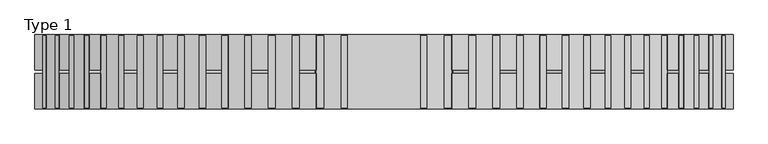
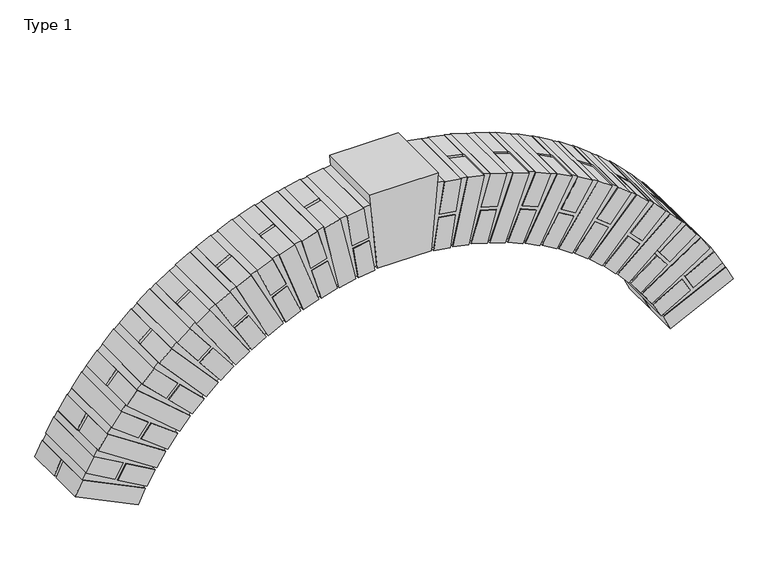
"""IFC4 building model written with IfcOpenShell, lengths in millimetres: proxy geometry, 00_GM_toog : Type 1."""

import ifcopenshell
import ifcopenshell.guid

model = None  # the IFC model being written
_history = None  # IfcOwnerHistory: only IFC2X3 demands one
_inside = {}  # id of a spatial element -> (the spatial element, [elements in it])
_under = {}  # id of a project, library or spatial element -> (it, [spatial elements below it])
_declared = {}  # id of a project -> (the project, [libraries it declares])
_typed = {}  # id of a type object -> (the type object, [elements of that type])
_made_of = {}  # id of a material, layer set ... -> (it, [elements and type objects made of it])


def new_model(schema):
    """Start an empty IFC model of exactly this schema.

    Asked for "IFC4X3", IfcOpenShell would pick the latest addendum, in which some entities
    have other attributes; the version numbers below select the first issue.
    IFC2X3 requires an IfcOwnerHistory on every rooted entity: one is made here for all.
    """
    global model, _history
    if schema == "IFC4X3":
        model = ifcopenshell.file(schema_version=(4, 3, 0, 0))
    else:
        model = ifcopenshell.file(schema=schema)
    _inside.clear()
    _under.clear()
    _declared.clear()
    _typed.clear()
    _made_of.clear()
    _history = None
    if model.schema == "IFC2X3":
        org = make("IfcOrganization", Name="unknown")
        user = make(
            "IfcPersonAndOrganization",
            ThePerson=make("IfcPerson", FamilyName="unknown"),
            TheOrganization=org,
        )
        app = make(
            "IfcApplication",
            ApplicationDeveloper=org,
            Version="unknown",
            ApplicationFullName="unknown",
            ApplicationIdentifier="unknown",
        )
        _history = make(
            "IfcOwnerHistory",
            OwningUser=user,
            OwningApplication=app,
            ChangeAction="ADDED",
            CreationDate=0,
        )
    return model


def make(cls, **values):
    """One entity of the class cls with the attributes given. An attribute that is None is left unset."""
    return model.create_entity(
        cls, **{name: value for name, value in values.items() if value is not None}
    )


def rooted(cls, **values):
    """An entity with a GlobalId (a new one), such as an element, a storey or a relation."""
    return make(cls, GlobalId=ifcopenshell.guid.new(), OwnerHistory=_history, **values)


def si_unit(unit_type, name, prefix=None):
    """IfcSIUnit, for example si_unit("LENGTHUNIT", "METRE", prefix="MILLI")."""
    return make("IfcSIUnit", UnitType=unit_type, Prefix=prefix, Name=name)


def assignment(units):
    """IfcUnitAssignment: the units of a project."""
    return None if units is None else make("IfcUnitAssignment", Units=units)


def point(xyz):
    """IfcCartesianPoint."""
    return None if xyz is None else make("IfcCartesianPoint", Coordinates=xyz)


def direction(xyz):
    """IfcDirection."""
    return None if xyz is None else make("IfcDirection", DirectionRatios=xyz)


def frame(location, z_axis=None, x_axis=None):
    """IfcAxis2Placement3D, a coordinate frame: its origin and axes. An axis left out is left unset."""
    return make(
        "IfcAxis2Placement3D",
        Location=point(location),
        Axis=direction(z_axis),
        RefDirection=direction(x_axis),
    )


def origin():
    """The frame at (0, 0, 0) with its axes left unset."""
    return frame((0.0, 0.0, 0.0))


def place(relative_to, where):
    """IfcLocalPlacement: puts the frame where relative to a parent placement (None: the world)."""
    return make(
        "IfcLocalPlacement", PlacementRelTo=relative_to, RelativePlacement=where
    )


def context(
    kind, dimensions, precision=None, world=None, true_north=None, identifier=None
):
    """IfcGeometricRepresentationContext, for example the 3D "Model" context."""
    return make(
        "IfcGeometricRepresentationContext",
        ContextIdentifier=identifier,
        ContextType=kind,
        CoordinateSpaceDimension=dimensions,
        Precision=precision,
        WorldCoordinateSystem=world,
        TrueNorth=true_north,
    )


def project(units=None, contexts=None):
    """IfcProject with its units and contexts."""
    return rooted(
        "IfcProject",
        Name="project",
        RepresentationContexts=contexts,
        UnitsInContext=assignment(units),
    )


def spatial(cls, under=None, at=None, **own):
    """A site, building, storey or space (cls), placed at a placement, below another one or the project."""
    s = rooted(cls, ObjectPlacement=at, **own)
    if under is not None:
        _under.setdefault(under.id(), (under, []))[1].append(s)
    return s


def polyline(points):
    """IfcPolyline through the points."""
    return make("IfcPolyline", Points=[point(p) for p in points])


def outline(outer, holes=None, kind="AREA"):
    """IfcArbitraryClosedProfileDef: a profile drawn as a closed curve; with holes, ...WithVoids."""
    if holes is None:
        return make("IfcArbitraryClosedProfileDef", ProfileType=kind, OuterCurve=outer)
    return make(
        "IfcArbitraryProfileDefWithVoids",
        ProfileType=kind,
        OuterCurve=outer,
        InnerCurves=holes,
    )


def extrude(swept, where, along, depth):
    """IfcExtrudedAreaSolid: the profile swept, set in the frame where, extruded along a direction by depth."""
    return make(
        "IfcExtrudedAreaSolid",
        SweptArea=swept,
        Position=where,
        ExtrudedDirection=direction(along),
        Depth=depth,
    )


def shape(context_of_items, identifier, shape_type, items):
    """IfcShapeRepresentation: the items that make up one representation, for example the "Body"."""
    return make(
        "IfcShapeRepresentation",
        ContextOfItems=context_of_items,
        RepresentationIdentifier=identifier,
        RepresentationType=shape_type,
        Items=items,
    )


def source(mapping_origin, context_of_items, identifier, shape_type, items):
    """IfcRepresentationMap: a shape defined once, which mapped items show again and again."""
    return make(
        "IfcRepresentationMap",
        MappingOrigin=mapping_origin,
        MappedRepresentation=shape(context_of_items, identifier, shape_type, items),
    )


def transform(
    local_origin,
    x_axis=None,
    y_axis=None,
    z_axis=None,
    scale=None,
    scale2=None,
    scale3=None,
    uniform=True,
):
    """IfcCartesianTransformationOperator3D, or its non-uniform kind. x_axis, y_axis, z_axis: its Axis1, 2, 3."""
    if uniform:
        return make(
            "IfcCartesianTransformationOperator3D",
            Axis1=direction(x_axis),
            Axis2=direction(y_axis),
            LocalOrigin=point(local_origin),
            Scale=scale,
            Axis3=direction(z_axis),
        )
    return make(
        "IfcCartesianTransformationOperator3DnonUniform",
        Axis1=direction(x_axis),
        Axis2=direction(y_axis),
        LocalOrigin=point(local_origin),
        Scale=scale,
        Axis3=direction(z_axis),
        Scale2=scale2,
        Scale3=scale3,
    )


def mapped(mapping_source, mapping_target):
    """IfcMappedItem: shows the shape of a source again, moved by a transform."""
    return make(
        "IfcMappedItem", MappingSource=mapping_source, MappingTarget=mapping_target
    )


def made_of(thing, what):
    """Note that an element or type object is made of a material, layer set ...; save() writes the relation."""
    if what is not None:
        _made_of.setdefault(what.id(), (what, []))[1].append(thing)
    return thing


def element(
    cls,
    number,
    at=None,
    inside=None,
    cuts=None,
    type_object=None,
    material=None,
    context=None,
    identifier="Body",
    shape_type=None,
    held_by="IfcProductDefinitionShape",
    body=None,
    shapes=None,
    **own,
):
    """One element of the class cls, such as IfcWall. Its Tag is "e" and its number.

    at: its placement. inside: the storey or other place that contains it. cuts: it is an
    opening in that element (IfcRelVoidsElement). A single representation is given by context,
    identifier, shape_type and body (its items); several are given by shapes. held_by: the class
    of the entity that holds the representations. save() writes the other relations.
    """
    e = rooted(cls, Tag="e%d" % number, ObjectPlacement=at, **own)
    if body is not None:
        shapes = [shape(context, identifier, shape_type, body)]
    if shapes is not None:
        e.Representation = make(held_by, Representations=shapes)
    if inside is not None:
        _inside.setdefault(inside.id(), (inside, []))[1].append(e)
    if cuts is not None:
        rooted(
            "IfcRelVoidsElement", RelatingBuildingElement=cuts, RelatedOpeningElement=e
        )
    if type_object is not None:
        _typed.setdefault(type_object.id(), (type_object, []))[1].append(e)
    return made_of(e, material)


def aggregate(whole, parts):
    """IfcRelAggregates: a whole, such as a stair, and the parts it consists of."""
    return rooted("IfcRelAggregates", RelatingObject=whole, RelatedObjects=parts)


def save(model, path):
    """Write the relations noted so far, then the file.

    IfcRelAggregates (storeys below a building ...), IfcRelContainedInSpatialStructure (elements
    in a storey), IfcRelDefinesByType, IfcRelAssociatesMaterial and IfcRelDeclares: one each for
    every whole, place, type object, material and project.
    """
    for whole, parts in _under.values():
        aggregate(whole, parts)
    for where, things in _inside.values():
        rooted(
            "IfcRelContainedInSpatialStructure",
            RelatedElements=things,
            RelatingStructure=where,
        )
    for kind, things in _typed.values():
        rooted("IfcRelDefinesByType", RelatedObjects=things, RelatingType=kind)
    for what, things in _made_of.values():
        rooted("IfcRelAssociatesMaterial", RelatedObjects=things, RelatingMaterial=what)
    for by, libraries in _declared.values():
        rooted("IfcRelDeclares", RelatingContext=by, RelatedDefinitions=libraries)
    model.write(path)


def type_1_0c07ca49(model_context):
    return source(origin(), model_context, "Body", "SweptSolid", [
        extrude(outline(polyline([(-45.6408721, 191.4818055), (-42.8894673, 170.9223699), (-141.6730221, 155.3721516), (-133.897913, 105.9803742), (-35.1143581, 121.5305924), (-31.8881677, 101.036053), (-232.700927, 82.4958258), (-234.4158083, 90.1571411), (-143.9996832, 104.390183), (-151.7747924, 153.7819605), (-244.0260363, 139.2600395), (-245.6920563, 146.7030645), (-45.6408721, 191.4818055)])), frame((0.0, 2.5, 0.0), z_axis=(0.0, 1.0, 0.0), x_axis=(0.0, 0.0, 1.0)), (0.0, 0.0, 1.0), 205.0),
        extrude(outline(polyline([(0.0, 50.0), (210.0, 50.0), (210.0, 0.0), (0.0, 0.0), (0.0, 50.0)])), frame((105.9803742, 210.0, -133.897913), z_axis=(0.15550218280693498, 0.0, 0.9878355486326045), x_axis=(0.0, -1.0, 0.0)), (0.0, 0.0, 1.0), 100.0),
        extrude(outline(polyline([(0.0, 50.0), (210.0, 50.0), (210.0, 0.0), (0.0, 0.0), (0.0, 50.0)])), frame((88.8399648, 210.0, -242.7832381), z_axis=(0.15550218280693498, 0.0, 0.9878355486326045), x_axis=(0.0, -1.0, 0.0)), (0.0, 0.0, 1.0), 100.0),
        extrude(outline(polyline([(210.0, 50.0), (210.0, 0.0), (110.0, 0.0), (110.0, 50.0), (210.0, 50.0)])), frame((194.4038505, 0.0, -261.4914261), z_axis=(0.2184312927282846, 0.0, 0.9758523302001438), x_axis=(0.0, 1.0, 0.0)), (0.0, 0.0, 1.0), 210.0),
        extrude(outline(polyline([(100.0, 50.0), (100.0, 0.0), (0.0, 0.0), (0.0, 50.0), (100.0, 50.0)])), frame((194.4038505, 0.0, -261.4914261), z_axis=(0.2184312927282846, 0.0, 0.9758523302001438), x_axis=(0.0, 1.0, 0.0)), (0.0, 0.0, 1.0), 210.0),
        extrude(outline(polyline([(-79.0011577, 328.483536), (-73.6449941, 308.4442712), (-169.6314476, 280.3978679), (-155.608246, 232.4046411), (-59.6217925, 260.4510444), (-53.8030292, 240.5368171), (-250.6000607, 196.486474), (-253.2799314, 203.8658279), (-165.42398, 229.5365694), (-179.4471816, 277.5297962), (-269.0862896, 251.3380319), (-271.689804, 258.5071292), (-79.0011577, 328.483536)])), frame((0.0, 2.5, 0.0), z_axis=(0.0, 1.0, 0.0), x_axis=(0.0, 0.0, 1.0)), (0.0, 0.0, 1.0), 205.0),
        extrude(outline(polyline([(0.0, 50.0), (210.0, 50.0), (210.0, 0.0), (0.0, 0.0), (0.0, 50.0)])), frame((232.4046411, 210.0, -155.608246), z_axis=(0.2804640326193317, 0.0, 0.9598645354459673), x_axis=(0.0, -1.0, 0.0)), (0.0, 0.0, 1.0), 100.0),
        extrude(outline(polyline([(0.0, 50.0), (210.0, 50.0), (210.0, 0.0), (0.0, 0.0), (0.0, 50.0)])), frame((201.4901661, 210.0, -261.4104336), z_axis=(0.2804640326193317, 0.0, 0.9598645354459673), x_axis=(0.0, -1.0, 0.0)), (0.0, 0.0, 1.0), 100.0),
        extrude(outline(polyline([(210.0, 50.0), (210.0, 0.0), (110.0, 0.0), (110.0, 50.0), (210.0, 50.0)])), frame((303.7977981, 0.0, -293.455382), z_axis=(0.34134584056160533, 0.0, 0.9399377730101558), x_axis=(0.0, 1.0, 0.0)), (0.0, 0.0, 1.0), 210.0),
        extrude(outline(polyline([(100.0, 50.0), (100.0, 0.0), (0.0, 0.0), (0.0, 50.0), (100.0, 50.0)])), frame((303.7977981, 0.0, -293.455382), z_axis=(0.34134584056160533, 0.0, 0.9399377730101558), x_axis=(0.0, 1.0, 0.0)), (0.0, 0.0, 1.0), 210.0),
        extrude(outline(polyline([(-129.5955556, 460.0988455), (-121.7224629, 440.9083522), (-213.3378444, 400.8256644), (-193.2965006, 355.0179737), (-101.681119, 395.1006614), (-93.3651981, 376.0932967), (-282.9194552, 307.2551682), (-286.5203712, 314.2315551), (-202.6652415, 350.9190515), (-222.7065854, 396.7267423), (-308.2636695, 359.294623), (-311.7619863, 366.072235), (-129.5955556, 460.0988455)])), frame((0.0, 2.5, 0.0), z_axis=(0.0, 1.0, 0.0), x_axis=(0.0, 0.0, 1.0)), (0.0, 0.0, 1.0), 205.0),
        extrude(outline(polyline([(0.0, 49.9999999), (210.0, 49.9999999), (210.0, 0.0), (0.0, 0.0), (0.0, 49.9999999)])), frame((355.0179737, 210.0, -193.2965006), z_axis=(0.40082687768196756, 0.0, 0.9161538157578809), x_axis=(0.0, -1.0, 0.0)), (0.0, 0.0, 1.0), 100.0),
        extrude(outline(polyline([(0.0, 50.0), (210.0, 50.0), (210.0, 0.0), (0.0, 0.0), (0.0, 50.0)])), frame((310.8363637, 210.0, -294.2806231), z_axis=(0.40082687768196756, 0.0, 0.9161538157578809), x_axis=(0.0, -1.0, 0.0)), (0.0, 0.0, 1.0), 100.0),
        extrude(outline(polyline([(210.0, 50.0), (210.0, 0.0), (110.0, 0.0), (110.0, 50.0), (210.0, 50.0)])), frame((408.2101175, 0.0, -339.136864), z_axis=(0.4586630534090749, 0.0, 0.8886102652104938), x_axis=(0.0, 1.0, 0.0)), (0.0, 0.0, 1.0), 210.0),
        extrude(outline(polyline([(100.0, 50.0), (100.0, 0.0), (0.0, 0.0), (0.0, 50.0), (100.0, 50.0)])), frame((408.2101175, 0.0, -339.136864), z_axis=(0.4586630534090749, 0.0, 0.8886102652104938), x_axis=(0.0, 1.0, 0.0)), (0.0, 0.0, 1.0), 210.0),
        extrude(outline(polyline([(-196.594427, 584.1695271), (-186.3335069, 566.142488), (-272.075522, 514.6807853), (-246.3446706, 471.8097777), (-160.6026555, 523.2714804), (-149.9259402, 505.482658), (-329.1291422, 412.9855408), (-333.5920562, 419.4445631), (-255.1127914, 466.5472186), (-280.8436427, 509.4182261), (-360.9157515, 461.3595579), (-365.2515057, 467.6345463), (-196.594427, 584.1695271)])), frame((0.0, 2.5, 0.0), z_axis=(0.0, 1.0, 0.0), x_axis=(0.0, 0.0, 1.0)), (0.0, 0.0, 1.0), 205.0),
        extrude(outline(polyline([(0.0, 50.0000001), (210.0, 50.0000001), (210.0, 0.0), (0.0, 0.0), (0.0, 50.0000001)])), frame((471.8097777, 210.0, -246.3446706), z_axis=(0.5146170271405577, 0.0, 0.8574201510210817), x_axis=(0.0, -1.0, 0.0)), (0.0, 0.0, 1.0), 100.0),
        extrude(outline(polyline([(0.0, 49.9999999), (210.0, 49.9999999), (210.0, 0.0), (0.0, 0.0), (0.0, 49.9999999)])), frame((415.0855159, 210.0, -340.8548065), z_axis=(0.5146170271405577, 0.0, 0.8574201510210817), x_axis=(0.0, -1.0, 0.0)), (0.0, 0.0, 1.0), 100.0),
        extrude(outline(polyline([(210.0, 50.0), (210.0, 0.0), (110.0, 0.0), (110.0, 50.0), (210.0, 50.0)])), frame((505.9286722, 0.0, -397.7867942), z_axis=(0.5684591822106966, 0.0, 0.8227114671379914), x_axis=(0.0, 1.0, 0.0)), (0.0, 0.0, 1.0), 210.0),
        extrude(outline(polyline([(100.0, 50.0), (100.0, 0.0), (0.0, 0.0), (0.0, 50.0), (100.0, 50.0)])), frame((505.9286722, 0.0, -397.7867942), z_axis=(0.5684591822106966, 0.0, 0.8227114671379914), x_axis=(0.0, 1.0, 0.0)), (0.0, 0.0, 1.0), 210.0),
        extrude(outline(polyline([(-278.8991351, 698.6610894), (-266.4186445, 682.093109), (-344.8813091, 620.0962521), (-313.8828807, 580.8649198), (-235.420216, 642.8617766), (-222.5577813, 626.5831948), (-388.4713826, 511.943842), (-393.7231125, 517.7795857), (-321.906603, 574.5250184), (-352.9050314, 613.7563507), (-426.1791551, 555.8591919), (-431.2812498, 561.5286604), (-278.8991351, 698.6610894)])), frame((0.0, 2.5, 0.0), z_axis=(0.0, 1.0, 0.0), x_axis=(0.0, 0.0, 1.0)), (0.0, 0.0, 1.0), 205.0),
        extrude(outline(polyline([(0.0, 50.0), (210.0, 50.0), (210.0, 0.0), (0.0, 0.0), (0.0, 50.0)])), frame((580.8649198, 210.0, -313.8828807), z_axis=(0.6199685681614698, 0.0, 0.784626646559889), x_axis=(0.0, -1.0, 0.0)), (0.0, 0.0, 1.0), 100.0),
        extrude(outline(polyline([(0.0, 50.0000001), (210.0, 50.0000001), (210.0, 0.0), (0.0, 0.0), (0.0, 50.0000001)])), frame((512.5281615, 210.0, -400.3692676), z_axis=(0.6199685681614698, 0.0, 0.784626646559889), x_axis=(0.0, -1.0, 0.0)), (0.0, 0.0, 1.0), 100.0),
        extrude(outline(polyline([(210.0, 50.0), (210.0, 0.0), (110.0, 0.0), (110.0, 50.0), (210.0, 50.0)])), frame((595.3510886, 0.0, -468.4434406), z_axis=(0.6689338074504708, 0.0, 0.7433219768376397), x_axis=(0.0, 1.0, 0.0)), (0.0, 0.0, 1.0), 210.0),
        extrude(outline(polyline([(100.0, 50.0), (100.0, 0.0), (0.0, 0.0), (0.0, 50.0), (100.0, 50.0)])), frame((595.3510886, 0.0, -468.4434406), z_axis=(0.6689338074504708, 0.0, 0.7433219768376397), x_axis=(0.0, 1.0, 0.0)), (0.0, 0.0, 1.0), 210.0),
        extrude(outline(polyline([(-375.1600602, 801.6961178), (-360.6646522, 786.8588753), (-430.5613481, 715.343479), (-394.8036499, 680.395131), (-324.9069541, 751.9105273), (-310.0697161, 737.4091197), (-459.9730918, 602.5073693), (-465.9275204, 607.6241406), (-401.951402, 673.0818479), (-437.7091002, 708.0301959), (-502.9837013, 641.243935), (-508.7684732, 646.2149166), (-375.1600602, 801.6961178)])), frame((0.0, 2.5, 0.0), z_axis=(0.0, 1.0, 0.0), x_axis=(0.0, 0.0, 1.0)), (0.0, 0.0, 1.0), 205.0),
        extrude(outline(polyline([(0.0, 100.0), (210.0, 100.0), (210.0, 0.0), (0.0, 0.0), (0.0, 100.0)])), frame((715.343479, 210.0, -430.5613481), z_axis=(-0.6989669587217563, 0.0, 0.7151539628746097), x_axis=(0.0, -1.0, 0.0)), (0.0, 0.0, 1.0), 50.0),
        extrude(outline(polyline([(0.0, 100.0), (210.0, 100.0), (210.0, 0.0), (0.0, 0.0), (0.0, 100.0)])), frame((636.5147996, 210.0, -507.6057961), z_axis=(-0.6989669587217563, 0.0, 0.7151539628746097), x_axis=(0.0, -1.0, 0.0)), (0.0, 0.0, 1.0), 50.0),
        extrude(outline(polyline([(0.0, 100.0), (210.0, 100.0), (210.0, 0.0), (0.0, 0.0), (0.0, 100.0)])), frame((675.0110323, 110.0, -549.9481866), z_axis=(-0.6517436105871354, 0.0, 0.7584393621502279), x_axis=(0.7584393621502279, 0.0, 0.6517436105871354)), (0.0, 0.0, 1.0), 50.0),
        extrude(outline(polyline([(0.0, 100.0), (210.0, 100.0), (210.0, 0.0), (0.0, 0.0), (0.0, 100.0)])), frame((675.0110323, 0.0, -549.9481866), z_axis=(-0.6517436105871354, 0.0, 0.7584393621502279), x_axis=(0.7584393621502279, 0.0, 0.6517436105871354)), (0.0, 0.0, 1.0), 50.0),
        extrude(outline(polyline([(-483.7987311, 891.5850605), (-467.5260991, 878.7218544), (-527.7106712, 798.8606168), (-487.7800524, 768.7683307), (-427.5954802, 848.6295684), (-411.0267377, 836.1431268), (-542.4617959, 683.1910761), (-549.0212836, 687.5049713), (-493.9346266, 760.6015881), (-533.8652454, 790.6938742), (-590.0699614, 716.1136617), (-596.4425527, 720.304643), (-483.7987311, 891.5850605)])), frame((0.0, 2.5, 0.0), z_axis=(0.0, 1.0, 0.0), x_axis=(0.0, 0.0, 1.0)), (0.0, 0.0, 1.0), 205.0),
        extrude(outline(polyline([(0.0, 99.9999999), (210.0, 99.9999999), (210.0, 0.0), (0.0, 0.0), (0.0, 99.9999999)])), frame((798.8606168, 210.0, -527.7106712), z_axis=(-0.6018457214896975, 0.0, 0.7986123762655734), x_axis=(0.0, -1.0, 0.0)), (0.0, 0.0, 1.0), 50.0),
        extrude(outline(polyline([(0.0, 100.0000001), (210.0, 100.0000001), (210.0, 0.0), (0.0, 0.0), (0.0, 100.0000001)])), frame((710.8326365, 210.0, -594.0498176), z_axis=(-0.6018457214896975, 0.0, 0.7986123762655734), x_axis=(0.0, -1.0, 0.0)), (0.0, 0.0, 1.0), 50.0),
        extrude(outline(polyline([(0.0, 100.0), (210.0, 100.0), (210.0, 0.0), (0.0, 0.0), (0.0, 100.0)])), frame((743.6022521, 110.0, -640.9645302), z_axis=(-0.5494780559199127, 0.0, 0.8355081484117753), x_axis=(0.8355081484117753, 0.0, 0.5494780559199127)), (0.0, 0.0, 1.0), 50.0),
        extrude(outline(polyline([(0.0, 100.0), (210.0, 100.0), (210.0, 0.0), (0.0, 0.0), (0.0, 100.0)])), frame((743.6022521, 0.0, -640.9645302), z_axis=(-0.5494780559199127, 0.0, 0.8355081484117753), x_axis=(0.8355081484117753, 0.0, 0.5494780559199127)), (0.0, 0.0, 1.0), 50.0),
        extrude(outline(polyline([(-603.0337079, 966.8539326), (-585.2506879, 956.175692), (-634.7362393, 869.2781649), (-591.2874757, 844.5353892), (-541.8019244, 931.4329163), (-523.7733689, 921.1661914), (-634.5848584, 752.6719241), (-641.6418437, 756.1122044), (-596.3479503, 835.6491039), (-639.7967139, 860.3918796), (-686.0099087, 779.24067), (-692.8658226, 782.582928), (-603.0337079, 966.8539326)])), frame((0.0, 2.5, 0.0), z_axis=(0.0, 1.0, 0.0), x_axis=(0.0, 0.0, 1.0)), (0.0, 0.0, 1.0), 205.0),
        extrude(outline(polyline([(0.0, 100.0000001), (210.0, 100.0000001), (210.0, 0.0), (0.0, 0.0), (0.0, 100.0000001)])), frame((869.2781649, 210.0, -634.7362393), z_axis=(-0.4948555135168874, 0.0, 0.8689752705007995), x_axis=(0.0, -1.0, 0.0)), (0.0, 0.0, 1.0), 50.0),
        extrude(outline(polyline([(0.0, 99.9999999), (210.0, 99.9999999), (210.0, 0.0), (0.0, 0.0), (0.0, 99.9999999)])), frame((773.4943526, 210.0, -689.2822652), z_axis=(-0.4948555135168874, 0.0, 0.8689752705007995), x_axis=(0.0, -1.0, 0.0)), (0.0, 0.0, 1.0), 50.0),
        extrude(outline(polyline([(0.0, 100.0), (210.0, 100.0), (210.0, 0.0), (0.0, 0.0), (0.0, 100.0)])), frame((800.0, 110.0, -740.0), z_axis=(-0.43820224719100825, 0.0, 0.8988764044943836), x_axis=(0.8988764044943836, 0.0, 0.43820224719100825)), (0.0, 0.0, 1.0), 50.0),
        extrude(outline(polyline([(0.0, 100.0), (210.0, 100.0), (210.0, 0.0), (0.0, 0.0), (0.0, 100.0)])), frame((800.0, 0.0, -740.0), z_axis=(-0.43820224719100825, 0.0, 0.8988764044943836), x_axis=(0.8988764044943836, 0.0, 0.43820224719100825)), (0.0, 0.0, 1.0), 50.0),
        extrude(outline(polyline([(-45.6408721, -191.4818055), (-245.6920563, -146.7030645), (-244.0260363, -139.2600395), (-151.7747924, -153.7819605), (-143.9996832, -104.390183), (-234.4158083, -90.1571411), (-232.700927, -82.4958258), (-31.8881677, -101.036053), (-35.1143581, -121.5305924), (-133.897913, -105.9803742), (-141.6730221, -155.3721516), (-42.8894673, -170.9223699), (-45.6408721, -191.4818055)])), frame((0.0, 2.5, 0.0), z_axis=(0.0, 1.0, 0.0), x_axis=(0.0, 0.0, 1.0)), (0.0, 0.0, 1.0), 205.0),
        extrude(outline(polyline([(0.0, -50.0), (0.0, 0.0), (210.0, 0.0), (210.0, -50.0), (0.0, -50.0)])), frame((-105.9803742, 210.0, -133.897913), z_axis=(-0.15550218280693498, 0.0, 0.9878355486326045), x_axis=(0.0, -1.0, 0.0)), (0.0, 0.0, 1.0), 100.0),
        extrude(outline(polyline([(0.0, -50.0), (0.0, 0.0), (210.0, 0.0), (210.0, -50.0), (0.0, -50.0)])), frame((-88.8399648, 210.0, -242.7832381), z_axis=(-0.15550218280693498, 0.0, 0.9878355486326045), x_axis=(0.0, -1.0, 0.0)), (0.0, 0.0, 1.0), 100.0),
        extrude(outline(polyline([(210.0, -50.0), (110.0, -50.0), (110.0, 0.0), (210.0, 0.0), (210.0, -50.0)])), frame((-194.4038505, 0.0, -261.4914261), z_axis=(-0.2184312927282846, 0.0, 0.9758523302001438), x_axis=(0.0, 1.0, 0.0)), (0.0, 0.0, 1.0), 210.0),
        extrude(outline(polyline([(100.0, -50.0), (0.0, -50.0), (0.0, 0.0), (100.0, 0.0), (100.0, -50.0)])), frame((-194.4038505, 0.0, -261.4914261), z_axis=(-0.2184312927282846, 0.0, 0.9758523302001438), x_axis=(0.0, 1.0, 0.0)), (0.0, 0.0, 1.0), 210.0),
        extrude(outline(polyline([(-79.0011577, -328.483536), (-271.689804, -258.5071292), (-269.0862896, -251.3380319), (-179.4471816, -277.5297962), (-165.42398, -229.5365694), (-253.2799314, -203.8658279), (-250.6000607, -196.486474), (-53.8030292, -240.5368171), (-59.6217925, -260.4510444), (-155.608246, -232.4046411), (-169.6314476, -280.3978679), (-73.6449941, -308.4442712), (-79.0011577, -328.483536)])), frame((0.0, 2.5, 0.0), z_axis=(0.0, 1.0, 0.0), x_axis=(0.0, 0.0, 1.0)), (0.0, 0.0, 1.0), 205.0),
        extrude(outline(polyline([(0.0, -50.0), (0.0, 0.0), (210.0, 0.0), (210.0, -50.0), (0.0, -50.0)])), frame((-232.4046411, 210.0, -155.608246), z_axis=(-0.2804640326193317, 0.0, 0.9598645354459673), x_axis=(0.0, -1.0, 0.0)), (0.0, 0.0, 1.0), 100.0),
        extrude(outline(polyline([(0.0, -50.0), (0.0, 0.0), (210.0, 0.0), (210.0, -50.0), (0.0, -50.0)])), frame((-201.4901661, 210.0, -261.4104336), z_axis=(-0.2804640326193317, 0.0, 0.9598645354459673), x_axis=(0.0, -1.0, 0.0)), (0.0, 0.0, 1.0), 100.0),
        extrude(outline(polyline([(210.0, -50.0), (110.0, -50.0), (110.0, 0.0), (210.0, 0.0), (210.0, -50.0)])), frame((-303.7977981, 0.0, -293.455382), z_axis=(-0.34134584056160533, 0.0, 0.9399377730101558), x_axis=(0.0, 1.0, 0.0)), (0.0, 0.0, 1.0), 210.0),
        extrude(outline(polyline([(100.0, -50.0), (0.0, -50.0), (0.0, 0.0), (100.0, 0.0), (100.0, -50.0)])), frame((-303.7977981, 0.0, -293.455382), z_axis=(-0.34134584056160533, 0.0, 0.9399377730101558), x_axis=(0.0, 1.0, 0.0)), (0.0, 0.0, 1.0), 210.0),
        extrude(outline(polyline([(-129.5955556, -460.0988455), (-311.7619863, -366.072235), (-308.2636695, -359.294623), (-222.7065854, -396.7267423), (-202.6652415, -350.9190515), (-286.5203712, -314.2315551), (-282.9194552, -307.2551682), (-93.3651981, -376.0932967), (-101.681119, -395.1006614), (-193.2965006, -355.0179737), (-213.3378444, -400.8256644), (-121.7224629, -440.9083522), (-129.5955556, -460.0988455)])), frame((0.0, 2.5, 0.0), z_axis=(0.0, 1.0, 0.0), x_axis=(0.0, 0.0, 1.0)), (0.0, 0.0, 1.0), 205.0),
        extrude(outline(polyline([(0.0, -49.9999999), (0.0, 0.0), (210.0, 0.0), (210.0, -49.9999999), (0.0, -49.9999999)])), frame((-355.0179737, 210.0, -193.2965006), z_axis=(-0.40082687768196756, 0.0, 0.9161538157578809), x_axis=(0.0, -1.0, 0.0)), (0.0, 0.0, 1.0), 100.0),
        extrude(outline(polyline([(0.0, -50.0), (0.0, 0.0), (210.0, 0.0), (210.0, -50.0), (0.0, -50.0)])), frame((-310.8363637, 210.0, -294.2806231), z_axis=(-0.40082687768196756, 0.0, 0.9161538157578809), x_axis=(0.0, -1.0, 0.0)), (0.0, 0.0, 1.0), 100.0),
        extrude(outline(polyline([(210.0, -50.0), (110.0, -50.0), (110.0, 0.0), (210.0, 0.0), (210.0, -50.0)])), frame((-408.2101175, 0.0, -339.136864), z_axis=(-0.4586630534090749, 0.0, 0.8886102652104938), x_axis=(0.0, 1.0, 0.0)), (0.0, 0.0, 1.0), 210.0),
        extrude(outline(polyline([(100.0, -50.0), (0.0, -50.0), (0.0, 0.0), (100.0, 0.0), (100.0, -50.0)])), frame((-408.2101175, 0.0, -339.136864), z_axis=(-0.4586630534090749, 0.0, 0.8886102652104938), x_axis=(0.0, 1.0, 0.0)), (0.0, 0.0, 1.0), 210.0),
        extrude(outline(polyline([(-196.594427, -584.1695271), (-365.2515057, -467.6345463), (-360.9157515, -461.3595579), (-280.8436427, -509.4182261), (-255.1127914, -466.5472186), (-333.5920562, -419.4445631), (-329.1291422, -412.9855408), (-149.9259402, -505.482658), (-160.6026555, -523.2714804), (-246.3446706, -471.8097777), (-272.075522, -514.6807853), (-186.3335069, -566.142488), (-196.594427, -584.1695271)])), frame((0.0, 2.5, 0.0), z_axis=(0.0, 1.0, 0.0), x_axis=(0.0, 0.0, 1.0)), (0.0, 0.0, 1.0), 205.0),
        extrude(outline(polyline([(0.0, -50.0000001), (0.0, 0.0), (210.0, 0.0), (210.0, -50.0000001), (0.0, -50.0000001)])), frame((-471.8097777, 210.0, -246.3446706), z_axis=(-0.5146170271405577, 0.0, 0.8574201510210817), x_axis=(0.0, -1.0, 0.0)), (0.0, 0.0, 1.0), 100.0),
        extrude(outline(polyline([(0.0, -49.9999999), (0.0, 0.0), (210.0, 0.0), (210.0, -49.9999999), (0.0, -49.9999999)])), frame((-415.0855159, 210.0, -340.8548065), z_axis=(-0.5146170271405577, 0.0, 0.8574201510210817), x_axis=(0.0, -1.0, 0.0)), (0.0, 0.0, 1.0), 100.0),
        extrude(outline(polyline([(210.0, -50.0), (110.0, -50.0), (110.0, 0.0), (210.0, 0.0), (210.0, -50.0)])), frame((-505.9286722, 0.0, -397.7867942), z_axis=(-0.5684591822106966, 0.0, 0.8227114671379914), x_axis=(0.0, 1.0, 0.0)), (0.0, 0.0, 1.0), 210.0),
        extrude(outline(polyline([(100.0, -50.0), (0.0, -50.0), (0.0, 0.0), (100.0, 0.0), (100.0, -50.0)])), frame((-505.9286722, 0.0, -397.7867942), z_axis=(-0.5684591822106966, 0.0, 0.8227114671379914), x_axis=(0.0, 1.0, 0.0)), (0.0, 0.0, 1.0), 210.0),
        extrude(outline(polyline([(-278.8991351, -698.6610894), (-431.2812498, -561.5286604), (-426.1791551, -555.8591919), (-352.9050314, -613.7563507), (-321.906603, -574.5250184), (-393.7231125, -517.7795857), (-388.4713826, -511.943842), (-222.5577813, -626.5831948), (-235.420216, -642.8617766), (-313.8828807, -580.8649198), (-344.8813091, -620.0962521), (-266.4186445, -682.093109), (-278.8991351, -698.6610894)])), frame((0.0, 2.5, 0.0), z_axis=(0.0, 1.0, 0.0), x_axis=(0.0, 0.0, 1.0)), (0.0, 0.0, 1.0), 205.0),
        extrude(outline(polyline([(0.0, -50.0), (0.0, 0.0), (210.0, 0.0), (210.0, -50.0), (0.0, -50.0)])), frame((-580.8649198, 210.0, -313.8828807), z_axis=(-0.6199685681614698, 0.0, 0.784626646559889), x_axis=(0.0, -1.0, 0.0)), (0.0, 0.0, 1.0), 100.0),
        extrude(outline(polyline([(0.0, -50.0000001), (0.0, 0.0), (210.0, 0.0), (210.0, -50.0000001), (0.0, -50.0000001)])), frame((-512.5281615, 210.0, -400.3692676), z_axis=(-0.6199685681614698, 0.0, 0.784626646559889), x_axis=(0.0, -1.0, 0.0)), (0.0, 0.0, 1.0), 100.0),
        extrude(outline(polyline([(210.0, -50.0), (110.0, -50.0), (110.0, 0.0), (210.0, 0.0), (210.0, -50.0)])), frame((-595.3510886, 0.0, -468.4434406), z_axis=(-0.6689338074504708, 0.0, 0.7433219768376397), x_axis=(0.0, 1.0, 0.0)), (0.0, 0.0, 1.0), 210.0),
        extrude(outline(polyline([(100.0, -50.0), (0.0, -50.0), (0.0, 0.0), (100.0, 0.0), (100.0, -50.0)])), frame((-595.3510886, 0.0, -468.4434406), z_axis=(-0.6689338074504708, 0.0, 0.7433219768376397), x_axis=(0.0, 1.0, 0.0)), (0.0, 0.0, 1.0), 210.0),
        extrude(outline(polyline([(-375.1600602, -801.6961178), (-508.7684732, -646.2149166), (-502.9837013, -641.243935), (-437.7091002, -708.0301959), (-401.951402, -673.0818479), (-465.9275204, -607.6241406), (-459.9730918, -602.5073693), (-310.0697161, -737.4091197), (-324.9069541, -751.9105273), (-394.8036499, -680.395131), (-430.5613481, -715.343479), (-360.6646522, -786.8588753), (-375.1600602, -801.6961178)])), frame((0.0, 2.5, 0.0), z_axis=(0.0, 1.0, 0.0), x_axis=(0.0, 0.0, 1.0)), (0.0, 0.0, 1.0), 205.0),
        extrude(outline(polyline([(0.0, -100.0), (0.0, 0.0), (210.0, 0.0), (210.0, -100.0), (0.0, -100.0)])), frame((-715.343479, 210.0, -430.5613481), z_axis=(0.6989669587217563, 0.0, 0.7151539628746097), x_axis=(0.0, -1.0, 0.0)), (0.0, 0.0, 1.0), 50.0),
        extrude(outline(polyline([(0.0, -100.0), (0.0, 0.0), (210.0, 0.0), (210.0, -100.0), (0.0, -100.0)])), frame((-636.5147996, 210.0, -507.6057961), z_axis=(0.6989669587217563, 0.0, 0.7151539628746097), x_axis=(0.0, -1.0, 0.0)), (0.0, 0.0, 1.0), 50.0),
        extrude(outline(polyline([(0.0, -100.0), (0.0, 0.0), (210.0, 0.0), (210.0, -100.0), (0.0, -100.0)])), frame((-675.0110323, 110.0, -549.9481866), z_axis=(0.6517436105871354, 0.0, 0.7584393621502279), x_axis=(-0.7584393621502279, 0.0, 0.6517436105871354)), (0.0, 0.0, 1.0), 50.0),
        extrude(outline(polyline([(0.0, -100.0), (0.0, 0.0), (210.0, 0.0), (210.0, -100.0), (0.0, -100.0)])), frame((-675.0110323, 0.0, -549.9481866), z_axis=(0.6517436105871354, 0.0, 0.7584393621502279), x_axis=(-0.7584393621502279, 0.0, 0.6517436105871354)), (0.0, 0.0, 1.0), 50.0),
        extrude(outline(polyline([(-483.7987311, -891.5850605), (-596.4425527, -720.304643), (-590.0699614, -716.1136617), (-533.8652454, -790.6938742), (-493.9346266, -760.6015881), (-549.0212836, -687.5049713), (-542.4617959, -683.1910761), (-411.0267377, -836.1431268), (-427.5954802, -848.6295684), (-487.7800524, -768.7683307), (-527.7106712, -798.8606168), (-467.5260991, -878.7218544), (-483.7987311, -891.5850605)])), frame((0.0, 2.5, 0.0), z_axis=(0.0, 1.0, 0.0), x_axis=(0.0, 0.0, 1.0)), (0.0, 0.0, 1.0), 205.0),
        extrude(outline(polyline([(0.0, -99.9999999), (0.0, 0.0), (210.0, 0.0), (210.0, -99.9999999), (0.0, -99.9999999)])), frame((-798.8606168, 210.0, -527.7106712), z_axis=(0.6018457214896975, 0.0, 0.7986123762655734), x_axis=(0.0, -1.0, 0.0)), (0.0, 0.0, 1.0), 50.0),
        extrude(outline(polyline([(0.0, -100.0000001), (0.0, 0.0), (210.0, 0.0), (210.0, -100.0000001), (0.0, -100.0000001)])), frame((-710.8326365, 210.0, -594.0498176), z_axis=(0.6018457214896975, 0.0, 0.7986123762655734), x_axis=(0.0, -1.0, 0.0)), (0.0, 0.0, 1.0), 50.0),
        extrude(outline(polyline([(0.0, -100.0), (0.0, 0.0), (210.0, 0.0), (210.0, -100.0), (0.0, -100.0)])), frame((-743.6022521, 110.0, -640.9645302), z_axis=(0.5494780559199127, 0.0, 0.8355081484117753), x_axis=(-0.8355081484117753, 0.0, 0.5494780559199127)), (0.0, 0.0, 1.0), 50.0),
        extrude(outline(polyline([(0.0, -100.0), (0.0, 0.0), (210.0, 0.0), (210.0, -100.0), (0.0, -100.0)])), frame((-743.6022521, 0.0, -640.9645302), z_axis=(0.5494780559199127, 0.0, 0.8355081484117753), x_axis=(-0.8355081484117753, 0.0, 0.5494780559199127)), (0.0, 0.0, 1.0), 50.0),
        extrude(outline(polyline([(-603.0337079, -966.8539326), (-692.8658226, -782.582928), (-686.0099087, -779.24067), (-639.7967139, -860.3918796), (-596.3479503, -835.6491039), (-641.6418437, -756.1122044), (-634.5848584, -752.6719241), (-523.7733689, -921.1661914), (-541.8019244, -931.4329163), (-591.2874757, -844.5353892), (-634.7362393, -869.2781649), (-585.2506879, -956.175692), (-603.0337079, -966.8539326)])), frame((0.0, 2.5, 0.0), z_axis=(0.0, 1.0, 0.0), x_axis=(0.0, 0.0, 1.0)), (0.0, 0.0, 1.0), 205.0),
        extrude(outline(polyline([(0.0, -100.0000001), (0.0, 0.0), (210.0, 0.0), (210.0, -100.0000001), (0.0, -100.0000001)])), frame((-869.2781649, 210.0, -634.7362393), z_axis=(0.4948555135168874, 0.0, 0.8689752705007995), x_axis=(0.0, -1.0, 0.0)), (0.0, 0.0, 1.0), 50.0),
        extrude(outline(polyline([(0.0, -99.9999999), (0.0, 0.0), (210.0, 0.0), (210.0, -99.9999999), (0.0, -99.9999999)])), frame((-773.4943526, 210.0, -689.2822652), z_axis=(0.4948555135168874, 0.0, 0.8689752705007995), x_axis=(0.0, -1.0, 0.0)), (0.0, 0.0, 1.0), 50.0),
        extrude(outline(polyline([(0.0, -100.0), (0.0, 0.0), (210.0, 0.0), (210.0, -100.0), (0.0, -100.0)])), frame((-800.0, 110.0, -740.0), z_axis=(0.43820224719100825, 0.0, 0.8988764044943836), x_axis=(-0.8988764044943836, 0.0, 0.43820224719100825)), (0.0, 0.0, 1.0), 50.0),
        extrude(outline(polyline([(0.0, -100.0), (0.0, 0.0), (210.0, 0.0), (210.0, -100.0), (0.0, -100.0)])), frame((-800.0, 0.0, -740.0), z_axis=(0.43820224719100825, 0.0, 0.8988764044943836), x_axis=(-0.8988764044943836, 0.0, 0.43820224719100825)), (0.0, 0.0, 1.0), 50.0),
        extrude(outline(polyline([(0.0, 102.7272727), (0.0, -102.7272727), (-240.0, -80.9090909), (-240.0, 80.9090909), (0.0, 102.7272727)])), frame((0.0, 0.0, 0.0), z_axis=(0.0, 1.0, 0.0), x_axis=(0.0, 0.0, 1.0)), (0.0, 0.0, 1.0), 210.0),
    ])


if __name__ == "__main__":
    model = new_model("IFC4")
    model_context = context("Model", 3, world=origin())
    ifc_project = project(units=[si_unit("LENGTHUNIT", "METRE", prefix="MILLI")], contexts=[model_context])
    site = spatial("IfcSite", under=ifc_project)
    building = spatial("IfcBuilding", under=site)
    placement = place(None, origin())
    type_1_shape = type_1_0c07ca49(model_context)
    element("IfcBuildingElementProxy", 1, Name="00_GM_toog : Type 1", ObjectType="00_GM_toog : Type 1", at=placement, inside=building, context=model_context, shape_type="MappedRepresentation", body=[
        mapped(type_1_shape, transform((0.0, 0.0, 0.0), x_axis=(1.0, 0.0, 0.0), y_axis=(0.0, 1.0, 0.0), z_axis=(0.0, 0.0, 1.0))),
    ])
    save(model, "model.ifc")

# Revit data of these elements
# Type "00_GM_toog : Type 1"
#   straal_hart_rollaag [instance default] = 1935 mm
#   straal_buitenlijn [instance default] = 2040 mm
#   straal [instance default] = 1830 mm
#   stootvoegbreedte_onderzijde [instance default] = 5 mm
#   offset [instance default] = -2070 mm
#   kop_voeg [instance default] = 55 mm
#   hoek_sluitsteen_half [instance default] = 2.80637°
#   hoek_kop [instance default] = 1.72149°
#   halve_breedte_tov_balk [instance default] = 200 mm
#   half_b [instance default] = 1800 mm
#   h_toog [instance default] = 1500 mm
#   h_steen [instance default] = 210 mm
#   h_sluitsteen [instance default] = 240 mm
#   h_kop [instance default] = 50 mm
#   dekdikte [instance default] = 240 mm
#   breedte [instance default] = 4000 mm
#   b_sluitsteen_bovenzijde [instance default] = 200 mm
#   apothema [instance default] = 330 mm
#   aantal_strekken [instance default] = 14
#   materiaal_voeg [instance default] = none
#   materiaal_strek [instance default] = none
#   materiaal_sluitsteen [instance default] = none
#   materiaal_koppen [instance default] = none
#   Default Elevation = 0
# Element 1 (IfcBuildingElementProxy, "00_GM_toog : Type 1")
#   straal_hart_rollaag = 995 mm
#   straal_buitenlijn = 1100 mm
#   straal = 890 mm
#   offset = -1130 mm
#   hoek_sluitsteen_half = 5.19443°
#   hoek_kop = 3.53625°
#   half_b = 800 mm
#   h_toog = 500 mm
#   breedte = 2000 mm
#   apothema = 390 mm
